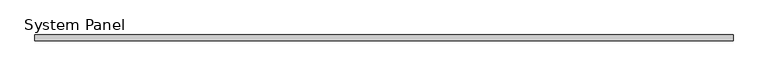
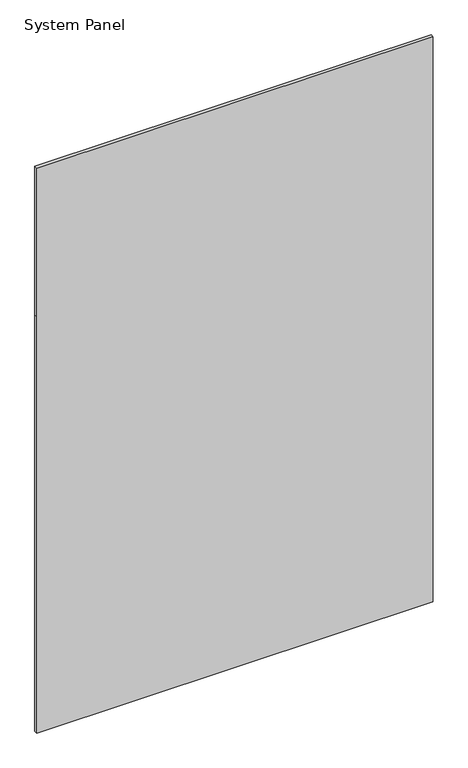
"""IFC4 building model written with IfcOpenShell, lengths in millimetres: plate geometry, System Panel : 로이복층유리_16."""

from ifc_helpers import new_model, si_unit, frame, origin, place, context, project, spatial, polyline, outline, extrude, source, transform, mapped, element, save


def system_panel_778a0f69(model_context):
    return source(origin(), model_context, "Body", "SweptSolid", [
        extrude(outline(polyline([(0.0, -980.9999999), (0.0, 980.9999999), (2177.5, 980.9999999), (2955.0, 980.9999999), (2955.0, -980.9999999), (2177.5, -980.9999999), (0.0, -980.9999999)])), frame((0.0, -8.0, 0.0), z_axis=(0.0, 1.0, 0.0), x_axis=(0.0, 0.0, 1.0)), (0.0, 0.0, 1.0), 16.0),
    ])


if __name__ == "__main__":
    model = new_model("IFC4")
    model_context = context("Model", 3, world=origin())
    ifc_project = project(units=[si_unit("LENGTHUNIT", "METRE", prefix="MILLI")], contexts=[model_context])
    site = spatial("IfcSite", under=ifc_project)
    building = spatial("IfcBuilding", under=site)
    placement = place(None, origin())
    system_panel_shape = system_panel_778a0f69(model_context)
    element("IfcPlate", 1, ObjectType="System Panel : 로이복층유리_16", at=placement, inside=building, context=model_context, shape_type="MappedRepresentation", body=[
        mapped(system_panel_shape, transform((0.0, 0.0, 0.0), x_axis=(1.0, 0.0, 0.0), y_axis=(0.0, 1.0, 0.0), z_axis=(0.0, 0.0, 1.0))),
    ])
    save(model, "model.ifc")

# Revit data of these elements
# Element 1 (IfcPlate, "System Panel : 로이복층유리_16")
#   Materials on its faces: "00_Glass_Glass"
# Materials
#   "00_Glass_Glass": class "Glass", colour RGB 218 227 224, transparency 0.85, Description = "Glass", Cost = 0, Image = none
